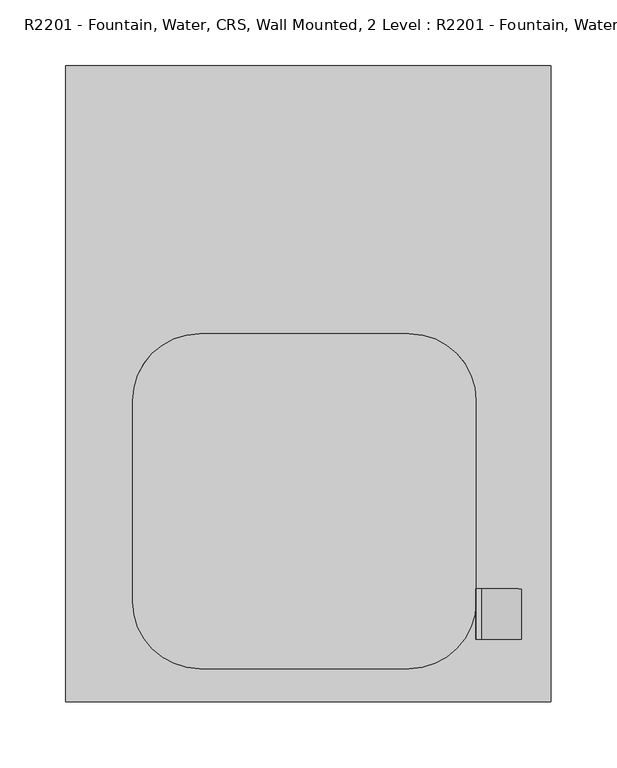
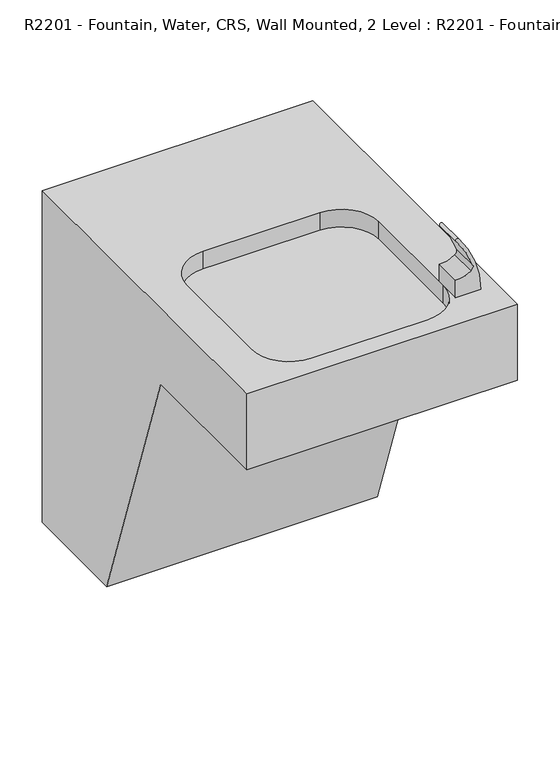
"""IFC4 building model written with IfcOpenShell, lengths in millimetres: proxy geometry, R2201 - Fountain, Water, CRS, Wall Mounted, 2 Level : R2201 - Fountain, Water, CRS, Wall Mounted, 2 Level."""

from ifc_helpers import new_model, si_unit, frame, origin, place, context, project, spatial, polyline, circle_curve, source, transform, mapped, element, save
from ifc_brep_helpers import plane_surface, cylinder_surface, revolved_surface, advanced_brep


def r2201_fountain_water_crs_wall_mounted_2_level_r2201_fountain_620c8a37(model_context):
    return source(origin(), model_context, "Body", "AdvancedBrep", [
        advanced_brep(
        [(184.15, -152.4, 152.4), (184.15, 0.0, 152.4), (184.15, 0.0, 630.2375), (184.15, -482.6, 630.2375), (184.15, -482.6, 520.7), (184.15, -279.4, 520.7), (-184.15, -152.4, 152.4), (-184.15, -279.4, 520.7), (-184.15, -482.6, 520.7), (-184.15, -482.6, 630.2375), (-184.15, 0.0, 630.2375), (-184.15, 0.0, 152.4), (-82.55, -203.2, 630.2375), (76.513502, -203.2, 630.2375), (127.313502, -254.0, 630.2375), (127.313502, -406.4, 630.2375), (76.513502, -457.2, 630.2375), (-82.55, -457.2, 630.2375), (-133.35, -406.4, 630.2375), (-133.35, -254.0, 630.2375), (76.513502, -203.2, 604.9069347), (-82.55, -203.2, 604.9069347), (-133.35, -254.0, 604.9069347), (-133.35, -406.4, 604.9069347), (-82.55, -457.2, 604.9069347), (76.513502, -457.2, 604.9069347), (127.313502, -406.4, 604.9069347), (127.313502, -254.0, 604.9069347)],
        [
            (0, 1),
            (1, 2),
            (2, 3),
            (3, 4),
            (4, 5),
            (5, 0),
            (6, 7),
            (7, 8),
            (8, 9),
            (9, 10),
            (10, 11),
            (11, 6),
            (0, 6),
            (11, 1),
            (10, 2),
            (9, 3),
            (12, 13),
            (13, 14, circle_curve(frame((76.513502, -254.0, 630.2375), z_axis=(0.0, 0.0, -1.0), x_axis=(0.0, -1.0, 0.0)), 50.8)),
            (14, 15),
            (15, 16, circle_curve(frame((76.513502, -406.4, 630.2375), z_axis=(0.0, 0.0, -1.0), x_axis=(0.0, -1.0, 0.0)), 50.8)),
            (16, 17),
            (17, 18, circle_curve(frame((-82.55, -406.4, 630.2375), z_axis=(0.0, 0.0, -1.0), x_axis=(0.0, -1.0, 0.0)), 50.8)),
            (18, 19),
            (19, 12, circle_curve(frame((-82.55, -254.0, 630.2375), z_axis=(0.0, 0.0, -1.0), x_axis=(0.0, -1.0, 0.0)), 50.8)),
            (8, 4),
            (7, 5),
            (20, 21),
            (21, 22, circle_curve(frame((-82.55, -254.0, 604.9069347), z_axis=(0.0, 0.0, 1.0), x_axis=(0.0, -1.0, 0.0)), 50.8)),
            (22, 23),
            (23, 24, circle_curve(frame((-82.55, -406.4, 604.9069347), z_axis=(0.0, 0.0, 1.0), x_axis=(0.0, -1.0, 0.0)), 50.8)),
            (24, 25),
            (25, 26, circle_curve(frame((76.513502, -406.4, 604.9069347), z_axis=(0.0, 0.0, 1.0), x_axis=(0.0, -1.0, 0.0)), 50.8)),
            (26, 27),
            (27, 20, circle_curve(frame((76.513502, -254.0, 604.9069347), z_axis=(0.0, 0.0, 1.0), x_axis=(0.0, -1.0, 0.0)), 50.8)),
            (20, 13),
            (12, 21),
            (19, 22),
            (18, 23),
            (17, 24),
            (16, 25),
            (15, 26),
            (14, 27),
        ],
        [
            plane_surface(frame((184.15, 0.0, 152.4), z_axis=(1.0, 0.0, 0.0), x_axis=(0.0, 1.0, 0.0))),
            plane_surface(frame((-184.15, 0.0, 152.4), z_axis=(-1.0, 0.0, 0.0), x_axis=(0.0, -1.0, 0.0))),
            plane_surface(frame((184.15, -152.4, 152.4), z_axis=(0.0, 0.0, -1.0), x_axis=(-1.0, 0.0, 0.0))),
            plane_surface(frame((184.15, 0.0, 152.4), z_axis=(0.0, 1.0, 0.0), x_axis=(-1.0, 0.0, 0.0))),
            plane_surface(frame((184.15, 0.0, 630.2375), z_axis=(0.0, 0.0, 1.0), x_axis=(-1.0, 0.0, 0.0))),
            plane_surface(frame((184.15, -482.6, 630.2375), z_axis=(0.0, -1.0, 0.0), x_axis=(-1.0, 0.0, 0.0))),
            plane_surface(frame((184.15, -482.6, 520.7), z_axis=(0.0, 0.0, -1.0), x_axis=(-1.0, 0.0, 0.0))),
            plane_surface(frame((184.15, -279.4, 520.7), z_axis=(0.0, -0.9453729816262746, -0.3259906833193972), x_axis=(-1.0, 0.0, 0.0))),
            plane_surface(frame((82.863502, -203.2, 604.9069347), z_axis=(0.0, 0.0, 1.0), x_axis=(1.0, 0.0, 0.0))),
            plane_surface(frame((76.513502, -203.2, 630.2375), z_axis=(0.0, -1.0, 0.0), x_axis=(0.0, 0.0, -1.0))),
            revolved_surface(polyline([(-82.55, -304.8, 630.2375), (-82.55, -304.8, 604.9069347)]), (-82.55, -254.0, 604.9069347), (0.0, 0.0, 1.0)),
            plane_surface(frame((-133.35, -254.0, 630.2375), z_axis=(1.0, 0.0, 0.0), x_axis=(0.0, 0.0, -1.0))),
            revolved_surface(polyline([(-82.55, -457.2, 630.2375), (-82.55, -457.2, 604.9069347)]), (-82.55, -406.4, 604.9069347), (0.0, 0.0, 1.0)),
            plane_surface(frame((-82.55, -457.2, 630.2375), z_axis=(0.0, 1.0, 0.0), x_axis=(0.0, 0.0, -1.0))),
            revolved_surface(polyline([(76.513502, -457.2, 630.2375), (76.513502, -457.2, 604.9069347)]), (76.513502, -406.4, 604.9069347), (0.0, 0.0, 1.0)),
            plane_surface(frame((127.313502, -406.4, 630.2375), z_axis=(-1.0, 0.0, 0.0), x_axis=(0.0, 0.0, -1.0))),
            revolved_surface(polyline([(76.513502, -304.8, 630.2375), (76.513502, -304.8, 604.9069347)]), (76.513502, -254.0, 604.9069347), (0.0, 0.0, 1.0)),
        ],
        [
            (0, [[1, 2, 3, 4, 5, 6]]),
            (1, [[7, 8, 9, 10, 11, 12]]),
            (2, [[-1, 13, -12, 14]]),
            (3, [[-2, -14, -11, 15]]),
            (4, [[-3, -15, -10, 16], [17, 18, 19, 20, 21, 22, 23, 24]]),
            (5, [[-4, -16, -9, 25]]),
            (6, [[-5, -25, -8, 26]]),
            (7, [[-6, -26, -7, -13]]),
            (8, [[27, 28, 29, 30, 31, 32, 33, 34]]),
            (9, [[-27, 35, -17, 36]]),
            (10, [[-28, -36, -24, 37]]),
            (11, [[-29, -37, -23, 38]]),
            (12, [[-30, -38, -22, 39]]),
            (13, [[-31, -39, -21, 40]]),
            (14, [[-32, -40, -20, 41]]),
            (15, [[-33, -41, -19, 42]]),
            (16, [[-34, -42, -18, -35]]),
        ],
    ),
        advanced_brep(
        [(131.5194093, -434.975, 713.776174), (128.2014816, -434.975, 711.1083712), (150.9349918, -434.975, 669.3013055), (148.6652265, -434.975, 662.1906851), (127.313502, -434.975, 655.6375), (127.313502, -434.975, 630.2375), (161.925, -434.975, 630.2375), (131.5194093, -396.875, 713.776174), (161.925, -396.875, 630.2375), (127.313502, -396.875, 630.2375), (127.313502, -396.875, 655.6375), (148.6652265, -396.875, 662.1906851), (150.9349918, -396.875, 669.3013055), (128.1944958, -396.875, 711.1027543)],
        [
            (0, 1, circle_curve(frame((129.8604454, -434.975, 712.4422726), z_axis=(0.0, -1.0, 0.0), x_axis=(1.0, 0.0, 0.0)), 2.1287212)),
            (1, 2, circle_curve(frame((24.0344482, -434.975, 627.3521456), z_axis=(0.0, 1.0, 0.0), x_axis=(1.0, 0.0, 0.0)), 133.6543302)),
            (2, 3, circle_curve(frame((144.9058684, -434.975, 667.308275), z_axis=(0.0, 1.0, 0.0), x_axis=(1.0, 0.0, 0.0)), 6.35)),
            (3, 4, circle_curve(frame((128.6007207, -434.975, 689.5043671), z_axis=(0.0, 1.0, 0.0), x_axis=(1.0, 0.0, 0.0)), 33.8913207)),
            (4, 5),
            (5, 6),
            (6, 0, circle_curve(frame((24.0344482, -434.975, 627.3521456), z_axis=(0.0, -1.0, 0.0), x_axis=(1.0, 0.0, 0.0)), 137.9207364)),
            (7, 8, circle_curve(frame((24.0344482, -396.875, 627.3521456), z_axis=(0.0, 1.0, 0.0), x_axis=(1.0, 0.0, 0.0)), 137.9207364)),
            (8, 9),
            (9, 10),
            (10, 11, circle_curve(frame((128.6007207, -396.875, 689.5043671), z_axis=(0.0, -1.0, 0.0), x_axis=(1.0, 0.0, 0.0)), 33.8913207)),
            (11, 12, circle_curve(frame((144.9058684, -396.875, 667.308275), z_axis=(0.0, -1.0, 0.0), x_axis=(1.0, 0.0, 0.0)), 6.35)),
            (12, 13, circle_curve(frame((24.0344482, -396.875, 627.3521456), z_axis=(0.0, -1.0, 0.0), x_axis=(1.0, 0.0, 0.0)), 133.6543302)),
            (13, 7, circle_curve(frame((129.8604454, -396.875, 712.4422726), z_axis=(0.0, 1.0, 0.0), x_axis=(1.0, 0.0, 0.0)), 2.1287212)),
            (0, 7),
            (13, 1),
            (12, 2),
            (11, 3),
            (10, 4),
            (9, 5),
            (8, 6),
        ],
        [
            plane_surface(frame((131.9891666, -434.975, 712.4422726), z_axis=(0.0, -1.0, 0.0), x_axis=(0.0, 0.0, 1.0))),
            plane_surface(frame((131.9891666, -396.875, 712.4422726), z_axis=(0.0, 1.0, 0.0), x_axis=(0.0, 0.0, -1.0))),
            cylinder_surface(frame((129.8604454, -396.875, 712.4422726), z_axis=(0.0, -1.0, 0.0), x_axis=(1.0, 0.0, 0.0)), 2.1287212),
            revolved_surface(polyline([(157.6887784, -396.875, 627.3521456), (157.6887784, -434.975, 627.3521456)]), (24.0344482, -396.875, 627.3521456), (0.0, 1.0, 0.0)),
            revolved_surface(polyline([(151.2558684, -396.875, 667.308275), (151.2558684, -434.975, 667.308275)]), (144.9058684, -396.875, 667.308275), (0.0, 1.0, 0.0)),
            revolved_surface(polyline([(162.4920414, -396.875, 689.5043671), (162.4920414, -434.975, 689.5043671)]), (128.6007207, -396.875, 689.5043671), (0.0, 1.0, 0.0)),
            plane_surface(frame((127.313502, -434.975, 655.6375), z_axis=(-1.0, 0.0, 0.0), x_axis=(0.0, 1.0, 0.0))),
            plane_surface(frame((127.313502, -434.975, 630.2375), z_axis=(0.0, 0.0, -1.0), x_axis=(0.0, 1.0, 0.0))),
            cylinder_surface(frame((24.0344482, -396.875, 627.3521456), z_axis=(0.0, -1.0, 0.0), x_axis=(1.0, 0.0, 0.0)), 137.9207364),
        ],
        [
            (0, [[1, 2, 3, 4, 5, 6, 7]]),
            (1, [[8, 9, 10, 11, 12, 13, 14]]),
            (2, [[-1, 15, -14, 16]]),
            (3, [[-2, -16, -13, 17]]),
            (4, [[-3, -17, -12, 18]]),
            (5, [[-4, -18, -11, 19]]),
            (6, [[-5, -19, -10, 20]]),
            (7, [[-6, -20, -9, 21]]),
            (8, [[-7, -21, -8, -15]]),
        ],
    ),
    ])


if __name__ == "__main__":
    model = new_model("IFC4")
    model_context = context("Model", 3, world=origin())
    ifc_project = project(units=[si_unit("LENGTHUNIT", "METRE", prefix="MILLI")], contexts=[model_context])
    site = spatial("IfcSite", under=ifc_project)
    building = spatial("IfcBuilding", under=site)
    placement = place(None, origin())
    r2201_fountain_water_crs_wall_mounted_2_level_r2201_fountain_shape = r2201_fountain_water_crs_wall_mounted_2_level_r2201_fountain_620c8a37(model_context)
    element("IfcBuildingElementProxy", 1, Name="R2201 - Fountain, Water, CRS, Wall Mounted, 2 Level : R2201 - Fountain, Water, CRS, Wall Mounted, 2 Level", ObjectType="R2201 - Fountain, Water, CRS, Wall Mounted, 2 Level : R2201 - Fountain, Water, CRS, Wall Mounted, 2 Level", at=placement, inside=building, context=model_context, shape_type="MappedRepresentation", body=[
        mapped(r2201_fountain_water_crs_wall_mounted_2_level_r2201_fountain_shape, transform((0.0, 0.0, 0.0), x_axis=(1.0, 0.0, 0.0), y_axis=(0.0, 1.0, 0.0), z_axis=(0.0, 0.0, 1.0))),
    ])
    save(model, "model.ifc")

# Revit data of these elements
# Type "R2201 - Fountain, Water, CRS, Wall Mounted, 2 Level : R2201 - Fountain, Water, CRS, Wall Mounted, 2 Level"
#   Youtube clip = ""
#   Uniclass 2.0 Description = ""
#   Uniclass 2.0 Code = ""
#   Uniclass 1.4 Description = ""
#   Uniclass 1.4 Code = ""
#   UNSPSC Code = ""
#   Technical description = ""
#   Region South America = "None"
#   Region Oceania = "None"
#   Region North America = "US"
#   Region Middle East = "None"
#   Region Europe = "None"
#   Region Asia = "None"
#   Region Antarctica = "None"
#   Region Africa = "None"
#   QR code = "http://bimobject.com/seps2bim/product/R2201"
#   Product group = ""
#   Product family = ""
#   Product data url = "https://bimobject.com/seps2bim/product/R2201"
#   Product certification = ""
#   Product SKU = "R2201"
#   Product Guid = "e3e6e1c2-7873-4cac-a932-e5ee46824a24"
#   OmniClass Description = ""
#   OmniClass Code = ""
#   NBS Reference Description = ""
#   NBS Reference Code = ""
#   Material secondary = ""
#   Material main = ""
#   Manufacturer name = "SEPS2BIM"
#   Manufacturer country = "United States"
#   Installation instructions = ""
#   IFC Classification = ""
#   EAN code = ""
#   Design country = "United States"
#   Description = "Drinking water fountain. This unit is a wall mounted, combination handicap and general public (2 level) dispenser. It contains an air cooled compressor with CRS wall protector. Specify with or without glass filler. It provides cool fresh drinking water, for hospitals and commercial office buildings."
#   Date of publishing = "2014-08-12"
#   COBIe Type Category = ""
#   BIMobject category = ""
#   Weight Net (Kg) = 0
#   Nominal width = 1020
#   Nominal height = 1040
#   Edition number = 1
# Element 1 (IfcBuildingElementProxy, "R2201 - Fountain, Water, CRS, Wall Mounted, 2 Level : R2201 - Fountain, Water, CRS, Wall Mounted, 2 Level")
#   Materials on its faces: "DRINKING FOUNTAIN"
# Materials
#   "DRINKING FOUNTAIN": class "Unassigned", colour RGB 247 247 247, transparency 0, Comments = "Rendering appearance not upgraded ", Cost = 0
